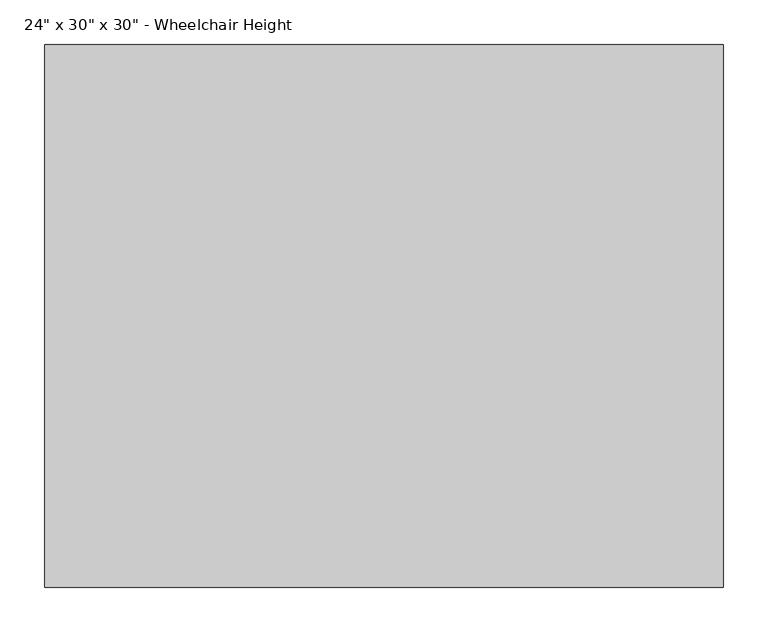
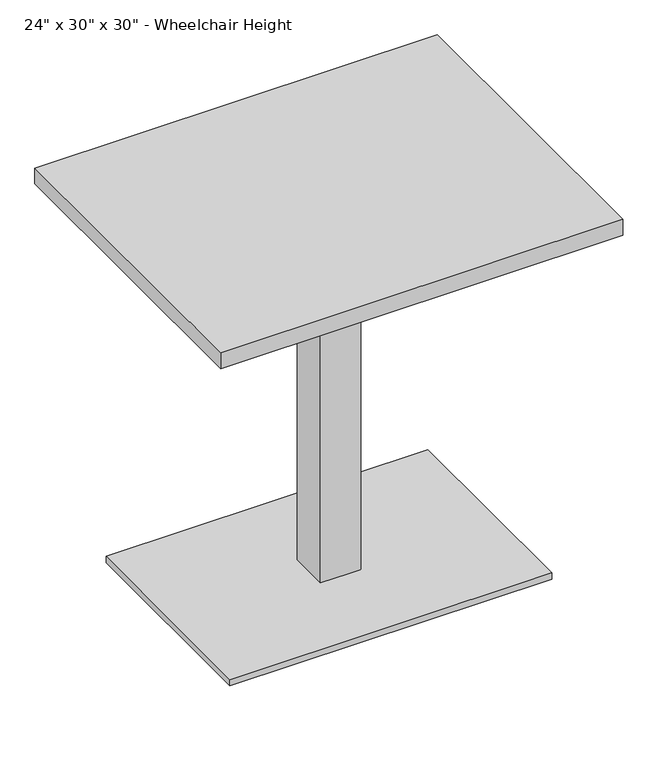
"""IFC4 building model written with IfcOpenShell, lengths in millimetres: furniture geometry."""

from ifc_helpers import new_model, si_unit, point, frame, frame_2d, origin, origin_with_axes, place, context, project, spatial, polyline, circle_curve, trimmed, segment, composite_curve, outline, extrude, source, transform, mapped, element, save


def furniture_cdcc8a0c(model_context):
    return source(origin(), model_context, "Body", "SweptSolid", [
        extrude(outline(composite_curve([segment(trimmed(circle_curve(frame_2d((107.7630735, 107.7630735)), 31.75), [point((77.0949285, 99.5455688))], [point((99.5455688, 77.0949285))], False, "CARTESIAN"), True, "CONTINUOUS"), segment(trimmed(circle_curve(frame_2d((97.9020678, 70.9612995)), 6.35), [point((99.5455688, 77.0949285))], [point((93.4119398, 75.4514275))], True, "CARTESIAN"), True, "CONTINUOUS"), segment(polyline([(93.4119398, 75.4514275), (17.9605122, 0.0), (93.4119398, -75.4514275)]), True, "CONTINUOUS"), segment(trimmed(circle_curve(frame_2d((97.9020678, -70.9612995)), 6.35), [point((93.4119398, -75.4514275))], [point((99.5455688, -77.0949285))], True, "CARTESIAN"), True, "CONTINUOUS"), segment(trimmed(circle_curve(frame_2d((107.7630735, -107.7630735)), 31.75), [point((99.5455688, -77.0949285))], [point((77.0949285, -99.5455688))], False, "CARTESIAN"), True, "CONTINUOUS"), segment(trimmed(circle_curve(frame_2d((70.9612995, -97.9020678)), 6.35), [point((77.0949285, -99.5455688))], [point((75.4514275, -93.4119398))], True, "CARTESIAN"), True, "CONTINUOUS"), segment(polyline([(75.4514275, -93.4119398), (0.0, -17.9605122), (-75.4514275, -93.4119398)]), True, "CONTINUOUS"), segment(trimmed(circle_curve(frame_2d((-70.9612995, -97.9020678)), 6.35), [point((-75.4514275, -93.4119398))], [point((-77.0949285, -99.5455688))], True, "CARTESIAN"), True, "CONTINUOUS"), segment(trimmed(circle_curve(frame_2d((-107.7630735, -107.7630735)), 31.75), [point((-77.0949285, -99.5455688))], [point((-99.5455688, -77.0949285))], False, "CARTESIAN"), True, "CONTINUOUS"), segment(trimmed(circle_curve(frame_2d((-97.9020678, -70.9612995)), 6.35), [point((-99.5455688, -77.0949285))], [point((-93.4119398, -75.4514275))], True, "CARTESIAN"), True, "CONTINUOUS"), segment(polyline([(-93.4119398, -75.4514275), (-17.9605122, 0.0), (-93.4119398, 75.4514275)]), True, "CONTINUOUS"), segment(trimmed(circle_curve(frame_2d((-97.9020678, 70.9612995)), 6.35), [point((-93.4119398, 75.4514275))], [point((-99.5455688, 77.0949285))], True, "CARTESIAN"), True, "CONTINUOUS"), segment(trimmed(circle_curve(frame_2d((-107.7630735, 107.7630735)), 31.75), [point((-99.5455688, 77.0949285))], [point((-77.0949285, 99.5455688))], False, "CARTESIAN"), True, "CONTINUOUS"), segment(trimmed(circle_curve(frame_2d((-70.9612995, 97.9020678)), 6.35), [point((-77.0949285, 99.5455688))], [point((-75.4514275, 93.4119398))], True, "CARTESIAN"), True, "CONTINUOUS"), segment(polyline([(-75.4514275, 93.4119398), (0.0, 17.9605122), (75.4514275, 93.4119398)]), True, "CONTINUOUS"), segment(trimmed(circle_curve(frame_2d((70.9612995, 97.9020678)), 6.35), [point((75.4514275, 93.4119398))], [point((77.0949285, 99.5455688))], True, "CARTESIAN"), True, "CONTINUOUS")], self_intersect=False)), frame((0.0, 0.0, 723.9), z_axis=(0.0, 0.0, 1.0), x_axis=(1.0, 0.0, 0.0)), (0.0, 0.0, 1.0), 6.35),
        extrude(outline(polyline([(-38.1, 38.1), (38.1, 38.1), (38.1, -38.1), (-38.1, -38.1), (-38.1, 38.1)])), frame((0.0, 0.0, 19.05), z_axis=(0.0, 0.0, 1.0), x_axis=(1.0, 0.0, 0.0)), (0.0, 0.0, 1.0), 704.85),
        extrude(outline(composite_curve([segment(trimmed(circle_curve(frame_2d((-276.4506403, -174.8506403)), 12.7), [point((-289.1506403, -174.8506403))], [point((-263.7506403, -174.8506403))], False, "CARTESIAN"), True, "CONTINUOUS"), segment(trimmed(circle_curve(frame_2d((-276.4506403, -174.8506403)), 12.7), [point((-263.7506403, -174.8506403))], [point((-289.1506403, -174.8506403))], False, "CARTESIAN"), True, "CONTINUOUS")], self_intersect=False)), origin_with_axes(), (0.0, 0.0, 1.0), 6.35),
        extrude(outline(composite_curve([segment(trimmed(circle_curve(frame_2d((-276.4506403, 174.8506403)), 12.7), [point((-289.1506403, 174.8506403))], [point((-263.7506403, 174.8506403))], False, "CARTESIAN"), True, "CONTINUOUS"), segment(trimmed(circle_curve(frame_2d((-276.4506403, 174.8506403)), 12.7), [point((-263.7506403, 174.8506403))], [point((-289.1506403, 174.8506403))], False, "CARTESIAN"), True, "CONTINUOUS")], self_intersect=False)), origin_with_axes(), (0.0, 0.0, 1.0), 6.35),
        extrude(outline(composite_curve([segment(trimmed(circle_curve(frame_2d((276.4506403, -174.8506403)), 12.7), [point((263.7506403, -174.8506403))], [point((289.1506403, -174.8506403))], False, "CARTESIAN"), True, "CONTINUOUS"), segment(trimmed(circle_curve(frame_2d((276.4506403, -174.8506403)), 12.7), [point((289.1506403, -174.8506403))], [point((263.7506403, -174.8506403))], False, "CARTESIAN"), True, "CONTINUOUS")], self_intersect=False)), origin_with_axes(), (0.0, 0.0, 1.0), 6.35),
        extrude(outline(composite_curve([segment(trimmed(circle_curve(frame_2d((276.4506403, 174.8506403)), 12.7), [point((263.7506403, 174.8506403))], [point((289.1506403, 174.8506403))], False, "CARTESIAN"), True, "CONTINUOUS"), segment(trimmed(circle_curve(frame_2d((276.4506403, 174.8506403)), 12.7), [point((289.1506403, 174.8506403))], [point((263.7506403, 174.8506403))], False, "CARTESIAN"), True, "CONTINUOUS")], self_intersect=False)), origin_with_axes(), (0.0, 0.0, 1.0), 6.35),
        extrude(outline(polyline([(304.8, 203.2), (304.8, -203.2), (-304.8, -203.2), (-304.8, 203.2), (304.8, 203.2)])), frame((0.0, 0.0, 6.35), z_axis=(0.0, 0.0, 1.0), x_axis=(1.0, 0.0, 0.0)), (0.0, 0.0, 1.0), 12.7),
        extrude(outline(polyline([(381.0, 304.8), (381.0, -304.8), (-381.0, -304.8), (-381.0, 304.8), (381.0, 304.8)])), frame((0.0, 0.0, 730.25), z_axis=(0.0, 0.0, 1.0), x_axis=(1.0, 0.0, 0.0)), (0.0, 0.0, 1.0), 31.75),
    ])


if __name__ == "__main__":
    model = new_model("IFC4")
    model_context = context("Model", 3, world=origin())
    ifc_project = project(units=[si_unit("LENGTHUNIT", "METRE", prefix="MILLI")], contexts=[model_context])
    site = spatial("IfcSite", under=ifc_project)
    building = spatial("IfcBuilding", under=site)
    placement = place(None, origin())
    furniture_shape = furniture_cdcc8a0c(model_context)
    element("IfcFurniture", 1, ObjectType="Falcon 7700 Series Pedestal Base : 24\" x 30\" x 30\" - Wheelchair Height", at=placement, inside=building, context=model_context, shape_type="MappedRepresentation", body=[
        mapped(furniture_shape, transform((0.0, 0.0, 0.0), x_axis=(1.0, 0.0, 0.0), y_axis=(0.0, 1.0, 0.0), z_axis=(0.0, 0.0, 1.0))),
    ])
    save(model, "model.ifc")

# Revit data of these elements
# Type "Falcon 7700 Series Pedestal Base : 24\" x 30\" x 30\" - Wheelchair Height"
#   URL = "http://www.commercialfurnituregroup.com/"
#   Product URL = "http://www.falconproducts.com/product/10525/Square-Table-Base.html"
#   Modeled By [instance default] = "http://www.therevitcollection.com"
#   Model Line = "Table Bases"
#   Model = "7700 Series"
#   Description = "Single Pedestal Table Base"
#   Brand = "Falcon"
#   Manufacturer = "Commercial Furniture Group Inc."
#   Assembly Code = "E2020200"
#   Table Width = 2' - 6"
#   Table Depth = 2' - 0"
#   Radius = 1' - 3"
#   Base Width = 2' - 0"
#   Table Thickness [instance default] = 0' - 1 1/4"
#   Height = 2' - 6"
#   Base Depth = 1' - 4"
#   Roundtop = no
#   RectangleTop = yes
#   Tabletop [instance default] = none
#   Table Base [instance default] = none
#   Type Comments = ""
#   Default Elevation = 0
# Element 1 (IfcFurniture, "Falcon 7700 Series Pedestal Base : 24\" x 30\" x 30\" - Wheelchair Height")
#   Tabletop = Metal - Aluminum
#   Table Base = Metal - Aluminum
#   Materials on its faces: "Metal - Aluminum"
# Materials
#   "Metal - Aluminum": class "Metal", colour RGB 247 247 247, transparency 0
